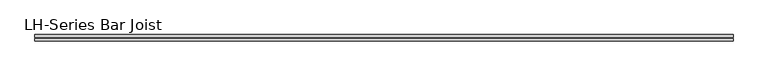
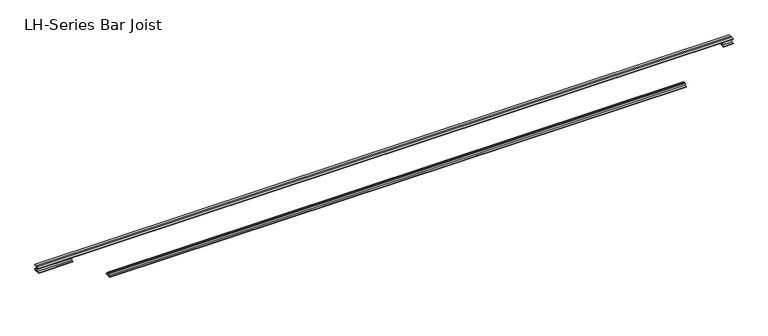
"""IFC4 building model written with IfcOpenShell, lengths in millimetres: beam geometry, LH-Series Bar Joist : 32LH-SP1."""

from ifc_helpers import new_model, si_unit, frame, origin, place, context, project, spatial, polyline, outline, extrude, source, transform, mapped, element, save


def lh_series_bar_joist_cdf094aa(model_context):
    return source(origin(), model_context, "Body", "SweptSolid", [
        extrude(outline(polyline([(12.7, 406.4), (76.2, 406.4), (76.2, 393.7), (25.4, 393.7), (25.4, 342.9), (12.7, 342.9), (12.7, 406.4)])), frame((-8397.875, 0.0, 0.0), z_axis=(1.0, 0.0, 0.0), x_axis=(0.0, 1.0, 0.0)), (0.0, 0.0, 1.0), 16224.25),
        extrude(outline(polyline([(-12.7, 406.4), (-12.7, 342.9), (-25.4, 342.9), (-25.4, 393.7), (-76.2, 393.7), (-76.2, 406.4), (-12.7, 406.4)])), frame((-8397.875, 0.0, 0.0), z_axis=(1.0, 0.0, 0.0), x_axis=(0.0, 1.0, 0.0)), (0.0, 0.0, 1.0), 16224.25),
        extrude(outline(polyline([(12.7, -406.4), (12.7, -342.9), (25.4, -342.9), (25.4, -393.7), (76.2, -393.7), (76.2, -406.4), (12.7, -406.4)])), frame((-6734.175, 0.0, 0.0), z_axis=(1.0, 0.0, 0.0), x_axis=(0.0, 1.0, 0.0)), (0.0, 0.0, 1.0), 13468.35),
        extrude(outline(polyline([(-12.7, -406.4), (-76.2, -406.4), (-76.2, -393.7), (-25.4, -393.7), (-25.4, -342.9), (-12.7, -342.9), (-12.7, -406.4)])), frame((-6734.175, 0.0, 0.0), z_axis=(1.0, 0.0, 0.0), x_axis=(0.0, 1.0, 0.0)), (0.0, 0.0, 1.0), 13468.35),
        extrude(outline(polyline([(12.7, 279.4), (12.7, 342.9), (25.4, 342.9), (25.4, 292.1), (76.2, 292.1), (76.2, 279.4), (12.7, 279.4)])), frame((7597.775, 0.0, 0.0), z_axis=(1.0, 0.0, 0.0), x_axis=(0.0, 1.0, 0.0)), (0.0, 0.0, 1.0), 228.6),
        extrude(outline(polyline([(-12.7, 279.4), (-76.2, 279.4), (-76.2, 292.1), (-25.4, 292.1), (-25.4, 342.9), (-12.7, 342.9), (-12.7, 279.4)])), frame((7597.775, 0.0, 0.0), z_axis=(1.0, 0.0, 0.0), x_axis=(0.0, 1.0, 0.0)), (0.0, 0.0, 1.0), 228.6),
        extrude(outline(polyline([(-12.7, 279.4), (-76.2, 279.4), (-76.2, 292.1), (-25.4, 292.1), (-25.4, 342.9), (-12.7, 342.9), (-12.7, 279.4)])), frame((-8397.875, 0.0, 0.0), z_axis=(1.0, 0.0, 0.0), x_axis=(0.0, 1.0, 0.0)), (0.0, 0.0, 1.0), 800.1),
        extrude(outline(polyline([(76.2, 279.4), (12.7, 279.4), (12.7, 342.9), (25.4, 342.9), (25.4, 292.1), (76.2, 292.1), (76.2, 279.4)])), frame((-8397.875, 0.0, 0.0), z_axis=(1.0, 0.0, 0.0), x_axis=(0.0, 1.0, 0.0)), (0.0, 0.0, 1.0), 800.1),
    ])


if __name__ == "__main__":
    model = new_model("IFC4")
    model_context = context("Model", 3, world=origin())
    ifc_project = project(units=[si_unit("LENGTHUNIT", "METRE", prefix="MILLI")], contexts=[model_context])
    site = spatial("IfcSite", under=ifc_project)
    building = spatial("IfcBuilding", under=site)
    placement = place(None, origin())
    lh_series_bar_joist_shape = lh_series_bar_joist_cdf094aa(model_context)
    element("IfcBeam", 1, ObjectType="LH-Series Bar Joist : 32LH-SP1", at=placement, inside=building, context=model_context, shape_type="MappedRepresentation", body=[
        mapped(lh_series_bar_joist_shape, transform((0.0, 0.0, 0.0), x_axis=(1.0, 0.0, 0.0), y_axis=(0.0, 1.0, 0.0), z_axis=(0.0, 0.0, 1.0))),
    ])
    save(model, "model.ifc")

# Revit data of these elements
# Type "LH-Series Bar Joist : 32LH-SP1"
#   Assembly Code = "B1010350"
#   Wt = 21
#   Web Thickness = 0' - 1"
#   Variable Panel [instance default] = 5' - 4"
#   Start Offset [instance default] = 0' - 0"
#   Start Extension [instance default] = 0' - 0"
#   Seat Length = 0' - 6"
#   Seat Depth = 0' - 5"
#   IntPanelWidth [instance default] = 5' - 4"
#   IntPanelArrayLength [instance default] = 21' - 4"
#   PanelAreaLength [instance default] = 32' - 0"
#   End Panel = 4' - 0"
#   End Offset [instance default] = 0' - 0"
#   End Extension [instance default] = 0' - 0"
#   Cord Leg = 0' - 2 1/2"
#   Chord Thickness = 0' - 0 1/2"
#   Length [instance default] = 40' - 0"
#   Depth = 2' - 8"
#   Vertical Member Visibility = yes
#   IntPanelArrayNum [instance default] = 4
#   Structural Material = none
# Element 1 (IfcBeam, "LH-Series Bar Joist : 32LH-SP1")
#   Variable Panel = 5' - 5 1/8"
#   Start Extension = 2' - 1 1/2"
#   IntPanelArrayLength = 32' - 0"
#   PanelAreaLength = 42' - 10 1/4"
#   End Extension = 0' - 3"
#   Length = 50' - 10 1/4"
#   IntPanelArrayNum = 6
